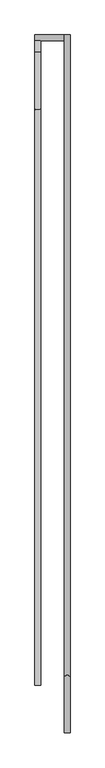
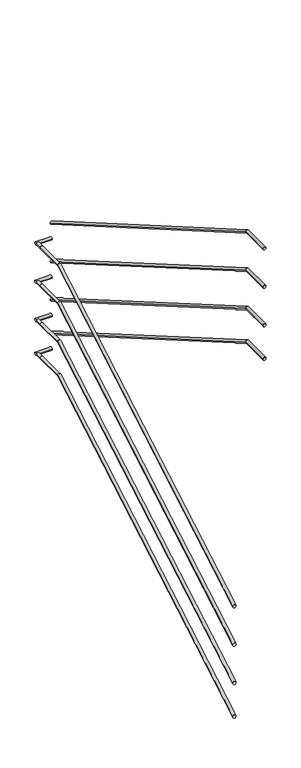
"""IFC4 building model written with IfcOpenShell, lengths in millimetres: railing geometry."""

from ifc_helpers import new_model, si_unit, frame, origin, place, context, project, spatial, circle_curve, ellipse_curve, source, transform, mapped, element, save
from ifc_brep_helpers import plane_surface, cylinder_surface, advanced_brep


def railing_01d63982(model_context):
    return source(origin(), model_context, "Body", "AdvancedBrep", [
        advanced_brep(
        [(52769.6, 12029.5208589, 12766.5366726), (52799.6, 12029.5208589, 12766.5366726), (52769.6, 15033.554313, 14508.0053416), (52799.6, 15033.554313, 14508.0053416), (52769.6, 15329.5208589, 14508.0053416), (52799.6, 15329.5208589, 14508.0053416)],
        [
            (0, 1, ellipse_curve(frame((52784.6, 12029.5208589, 12766.5366726), z_axis=(0.0, -1.0, 0.0), x_axis=(0.0, 0.0, -1.0)), 17.3382342, 15.0)),
            (1, 0, ellipse_curve(frame((52784.6, 12029.5208589, 12766.5366726), z_axis=(0.0, -1.0, 0.0), x_axis=(0.0, 0.0, -1.0)), 17.3382342, 15.0)),
            (0, 2),
            (2, 3, ellipse_curve(frame((52784.6, 15033.554313, 14508.0053416), z_axis=(0.0, -0.9656966401166088, -0.25967286971782944), x_axis=(0.0, 0.25967286971782905, -0.9656966401166089)), 15.5328282, 15.0)),
            (3, 1),
            (3, 2, ellipse_curve(frame((52784.6, 15033.554313, 14508.0053416), z_axis=(0.0, -0.9656966401166088, -0.25967286971782944), x_axis=(0.0, 0.25967286971782905, -0.9656966401166089)), 15.5328282, 15.0)),
            (4, 5, circle_curve(frame((52784.6, 15329.5208589, 14508.0053416), z_axis=(0.0, 1.0, 0.0), x_axis=(1.0, 0.0, 0.0)), 15.0)),
            (5, 4, circle_curve(frame((52784.6, 15329.5208589, 14508.0053416), z_axis=(0.0, 1.0, 0.0), x_axis=(1.0, 0.0, 0.0)), 15.0)),
            (2, 4),
            (5, 3),
        ],
        [
            plane_surface(frame((52784.6, 12029.5208589, 12783.8749068), z_axis=(0.0, -1.0, 0.0), x_axis=(0.0, 0.0, 1.0))),
            cylinder_surface(frame((52784.6, 12037.0438154, 12770.8978068), z_axis=(0.0, -0.8651400014650144, -0.5015304356318916), x_axis=(1.0, 0.0, 0.0)), 15.0),
            plane_surface(frame((52784.6, 15329.5208589, 14523.0053416), z_axis=(0.0, 1.0, 0.0), x_axis=(0.0, 0.0, 1.0))),
            cylinder_surface(frame((52784.6, 15029.5208589, 14508.0053416), z_axis=(0.0, -1.0, 0.0), x_axis=(1.0, 0.0, 0.0)), 15.0),
        ],
        [
            (0, [[1, 2]]),
            (1, [[-1, 3, 4, 5]]),
            (1, [[-2, -5, 6, -3]]),
            (2, [[7, 8]]),
            (3, [[-4, 9, -8, 10]]),
            (3, [[-6, -10, -7, -9]]),
        ],
    ),
        advanced_brep(
        [(52769.6, 15329.5208589, 14508.0053416), (52799.6, 15329.5208589, 14508.0053416), (52769.6, 15389.9208589, 14508.0053416), (52799.6, 15389.9208589, 14508.0053416)],
        [
            (0, 1, circle_curve(frame((52784.6, 15329.5208589, 14508.0053416), z_axis=(0.0, -1.0, 0.0), x_axis=(1.0, 0.0, 0.0)), 15.0)),
            (1, 0, circle_curve(frame((52784.6, 15329.5208589, 14508.0053416), z_axis=(0.0, -1.0, 0.0), x_axis=(1.0, 0.0, 0.0)), 15.0)),
            (2, 3, circle_curve(frame((52784.6, 15389.9208589, 14508.0053416), z_axis=(0.0, 1.0, 0.0), x_axis=(1.0, 0.0, 0.0)), 15.0)),
            (3, 2, circle_curve(frame((52784.6, 15389.9208589, 14508.0053416), z_axis=(0.0, 1.0, 0.0), x_axis=(1.0, 0.0, 0.0)), 15.0)),
            (0, 2),
            (3, 1),
        ],
        [
            plane_surface(frame((52784.6, 15329.5208589, 14523.0053416), z_axis=(0.0, -1.0, 0.0), x_axis=(0.0, 0.0, 1.0))),
            plane_surface(frame((52784.6, 15389.9208589, 14523.0053416), z_axis=(0.0, 1.0, 0.0), x_axis=(0.0, 0.0, 1.0))),
            cylinder_surface(frame((52784.6, 15329.5208589, 14508.0053416), z_axis=(0.0, -1.0, 0.0), x_axis=(1.0, 0.0, 0.0)), 15.0),
        ],
        [
            (0, [[1, 2]]),
            (1, [[3, 4]]),
            (2, [[-1, 5, -4, 6]]),
            (2, [[-2, -6, -3, -5]]),
        ],
    ),
        advanced_brep(
        [(52769.6, 15419.9208589, 14508.0053416), (52769.6, 15389.9208589, 14508.0053416), (52922.635546, 15419.9208589, 14508.0053416), (52922.635546, 15389.9208589, 14508.0053416)],
        [
            (0, 1, circle_curve(frame((52769.6, 15404.9208589, 14508.0053416), z_axis=(-1.0, 0.0, 0.0), x_axis=(0.0, -1.0, 0.0)), 15.0)),
            (1, 0, circle_curve(frame((52769.6, 15404.9208589, 14508.0053416), z_axis=(-1.0, 0.0, 0.0), x_axis=(0.0, -1.0, 0.0)), 15.0)),
            (2, 3, circle_curve(frame((52922.635546, 15404.9208589, 14508.0053416), z_axis=(1.0, 0.0, 0.0), x_axis=(0.0, -1.0, 0.0)), 15.0)),
            (3, 2, circle_curve(frame((52922.635546, 15404.9208589, 14508.0053416), z_axis=(1.0, 0.0, 0.0), x_axis=(0.0, -1.0, 0.0)), 15.0)),
            (0, 2),
            (3, 1),
        ],
        [
            plane_surface(frame((52769.6, 15404.9208589, 14523.0053416), z_axis=(-1.0, 0.0, 0.0), x_axis=(0.0, 1.0, 0.0))),
            plane_surface(frame((52922.635546, 15404.9208589, 14523.0053416), z_axis=(1.0, 0.0, 0.0), x_axis=(0.0, 1.0, 0.0))),
            cylinder_surface(frame((52769.6, 15404.9208589, 14508.0053416), z_axis=(-1.0, 0.0, 0.0), x_axis=(0.0, -1.0, 0.0)), 15.0),
        ],
        [
            (0, [[1, 2]]),
            (1, [[3, 4]]),
            (2, [[-1, 5, -4, 6]]),
            (2, [[-2, -6, -3, -5]]),
        ],
    ),
        advanced_brep(
        [(52952.635546, 15419.9208589, 14656.159861), (52922.635546, 15419.9208589, 14656.159861), (52952.635546, 12075.4874048, 16594.9618634), (52922.635546, 12075.4874048, 16594.9618634), (52952.635546, 11779.5208589, 16594.9618634), (52922.635546, 11779.5208589, 16594.9618634)],
        [
            (0, 1, ellipse_curve(frame((52937.635546, 15419.9208589, 14656.159861), z_axis=(0.0, 1.0, 0.0), x_axis=(0.0, 0.0, -1.0)), 17.3382342, 15.0)),
            (1, 0, ellipse_curve(frame((52937.635546, 15419.9208589, 14656.159861), z_axis=(0.0, 1.0, 0.0), x_axis=(0.0, 0.0, -1.0)), 17.3382342, 15.0)),
            (0, 2),
            (2, 3, ellipse_curve(frame((52937.635546, 12075.4874048, 16594.9618634), z_axis=(0.0, 0.9656966401166087, -0.2596728697178297), x_axis=(0.0, -0.259672869717829, -0.9656966401166089)), 15.5328282, 15.0)),
            (3, 1),
            (3, 2, ellipse_curve(frame((52937.635546, 12075.4874048, 16594.9618634), z_axis=(0.0, 0.9656966401166087, -0.2596728697178297), x_axis=(0.0, -0.259672869717829, -0.9656966401166089)), 15.5328282, 15.0)),
            (4, 5, circle_curve(frame((52937.635546, 11779.5208589, 16594.9618634), z_axis=(0.0, -1.0, 0.0), x_axis=(-1.0, 0.0, 0.0)), 15.0)),
            (5, 4, circle_curve(frame((52937.635546, 11779.5208589, 16594.9618634), z_axis=(0.0, -1.0, 0.0), x_axis=(-1.0, 0.0, 0.0)), 15.0)),
            (2, 4),
            (5, 3),
        ],
        [
            plane_surface(frame((52937.635546, 15419.9208589, 14673.4980953), z_axis=(0.0, 1.0, 0.0), x_axis=(0.0, 0.0, -1.0))),
            cylinder_surface(frame((52937.635546, 15412.3979024, 14660.5209952), z_axis=(0.0, 0.865140001465014, -0.5015304356318923), x_axis=(-1.0, 0.0, 0.0)), 15.0),
            plane_surface(frame((52937.635546, 11779.5208589, 16609.9618634), z_axis=(0.0, -1.0, 0.0), x_axis=(0.0, 0.0, -1.0))),
            cylinder_surface(frame((52937.635546, 12079.5208589, 16594.9618634), z_axis=(0.0, 1.0, 0.0), x_axis=(-1.0, 0.0, 0.0)), 15.0),
        ],
        [
            (0, [[1, 2]]),
            (1, [[-1, 3, 4, 5]]),
            (1, [[-2, -5, 6, -3]]),
            (2, [[7, 8]]),
            (3, [[-4, 9, -8, 10]]),
            (3, [[-6, -10, -7, -9]]),
        ],
    ),
        advanced_brep(
        [(52769.6, 12029.5208589, 11966.5366726), (52799.6, 12029.5208589, 11966.5366726), (52769.6, 15033.554313, 13708.0053416), (52799.6, 15033.554313, 13708.0053416), (52769.6, 15329.5208589, 13708.0053416), (52799.6, 15329.5208589, 13708.0053416)],
        [
            (0, 1, ellipse_curve(frame((52784.6, 12029.5208589, 11966.5366726), z_axis=(0.0, -1.0, 0.0), x_axis=(0.0, 0.0, -1.0)), 17.3382342, 15.0)),
            (1, 0, ellipse_curve(frame((52784.6, 12029.5208589, 11966.5366726), z_axis=(0.0, -1.0, 0.0), x_axis=(0.0, 0.0, -1.0)), 17.3382342, 15.0)),
            (0, 2),
            (2, 3, ellipse_curve(frame((52784.6, 15033.554313, 13708.0053416), z_axis=(0.0, -0.9656966401166088, -0.25967286971782944), x_axis=(0.0, 0.25967286971782905, -0.9656966401166089)), 15.5328282, 15.0)),
            (3, 1),
            (3, 2, ellipse_curve(frame((52784.6, 15033.554313, 13708.0053416), z_axis=(0.0, -0.9656966401166088, -0.25967286971782944), x_axis=(0.0, 0.25967286971782905, -0.9656966401166089)), 15.5328282, 15.0)),
            (4, 5, circle_curve(frame((52784.6, 15329.5208589, 13708.0053416), z_axis=(0.0, 1.0, 0.0), x_axis=(1.0, 0.0, 0.0)), 15.0)),
            (5, 4, circle_curve(frame((52784.6, 15329.5208589, 13708.0053416), z_axis=(0.0, 1.0, 0.0), x_axis=(1.0, 0.0, 0.0)), 15.0)),
            (2, 4),
            (5, 3),
        ],
        [
            plane_surface(frame((52784.6, 12029.5208589, 11983.8749068), z_axis=(0.0, -1.0, 0.0), x_axis=(0.0, 0.0, 1.0))),
            cylinder_surface(frame((52784.6, 12037.0438154, 11970.8978068), z_axis=(0.0, -0.8651400014650144, -0.5015304356318916), x_axis=(1.0, 0.0, 0.0)), 15.0),
            plane_surface(frame((52784.6, 15329.5208589, 13723.0053416), z_axis=(0.0, 1.0, 0.0), x_axis=(0.0, 0.0, 1.0))),
            cylinder_surface(frame((52784.6, 15029.5208589, 13708.0053416), z_axis=(0.0, -1.0, 0.0), x_axis=(1.0, 0.0, 0.0)), 15.0),
        ],
        [
            (0, [[1, 2]]),
            (1, [[-1, 3, 4, 5]]),
            (1, [[-2, -5, 6, -3]]),
            (2, [[7, 8]]),
            (3, [[-4, 9, -8, 10]]),
            (3, [[-6, -10, -7, -9]]),
        ],
    ),
        advanced_brep(
        [(52769.6, 15329.5208589, 13708.0053416), (52799.6, 15329.5208589, 13708.0053416), (52769.6, 15389.9208589, 13708.0053416), (52799.6, 15389.9208589, 13708.0053416)],
        [
            (0, 1, circle_curve(frame((52784.6, 15329.5208589, 13708.0053416), z_axis=(0.0, -1.0, 0.0), x_axis=(1.0, 0.0, 0.0)), 15.0)),
            (1, 0, circle_curve(frame((52784.6, 15329.5208589, 13708.0053416), z_axis=(0.0, -1.0, 0.0), x_axis=(1.0, 0.0, 0.0)), 15.0)),
            (2, 3, circle_curve(frame((52784.6, 15389.9208589, 13708.0053416), z_axis=(0.0, 1.0, 0.0), x_axis=(1.0, 0.0, 0.0)), 15.0)),
            (3, 2, circle_curve(frame((52784.6, 15389.9208589, 13708.0053416), z_axis=(0.0, 1.0, 0.0), x_axis=(1.0, 0.0, 0.0)), 15.0)),
            (0, 2),
            (3, 1),
        ],
        [
            plane_surface(frame((52784.6, 15329.5208589, 13723.0053416), z_axis=(0.0, -1.0, 0.0), x_axis=(0.0, 0.0, 1.0))),
            plane_surface(frame((52784.6, 15389.9208589, 13723.0053416), z_axis=(0.0, 1.0, 0.0), x_axis=(0.0, 0.0, 1.0))),
            cylinder_surface(frame((52784.6, 15329.5208589, 13708.0053416), z_axis=(0.0, -1.0, 0.0), x_axis=(1.0, 0.0, 0.0)), 15.0),
        ],
        [
            (0, [[1, 2]]),
            (1, [[3, 4]]),
            (2, [[-1, 5, -4, 6]]),
            (2, [[-2, -6, -3, -5]]),
        ],
    ),
        advanced_brep(
        [(52769.6, 15419.9208589, 13708.0053416), (52769.6, 15389.9208589, 13708.0053416), (52922.635546, 15419.9208589, 13708.0053416), (52922.635546, 15389.9208589, 13708.0053416)],
        [
            (0, 1, circle_curve(frame((52769.6, 15404.9208589, 13708.0053416), z_axis=(-1.0, 0.0, 0.0), x_axis=(0.0, -1.0, 0.0)), 15.0)),
            (1, 0, circle_curve(frame((52769.6, 15404.9208589, 13708.0053416), z_axis=(-1.0, 0.0, 0.0), x_axis=(0.0, -1.0, 0.0)), 15.0)),
            (2, 3, circle_curve(frame((52922.635546, 15404.9208589, 13708.0053416), z_axis=(1.0, 0.0, 0.0), x_axis=(0.0, -1.0, 0.0)), 15.0)),
            (3, 2, circle_curve(frame((52922.635546, 15404.9208589, 13708.0053416), z_axis=(1.0, 0.0, 0.0), x_axis=(0.0, -1.0, 0.0)), 15.0)),
            (0, 2),
            (3, 1),
        ],
        [
            plane_surface(frame((52769.6, 15404.9208589, 13723.0053416), z_axis=(-1.0, 0.0, 0.0), x_axis=(0.0, 1.0, 0.0))),
            plane_surface(frame((52922.635546, 15404.9208589, 13723.0053416), z_axis=(1.0, 0.0, 0.0), x_axis=(0.0, 1.0, 0.0))),
            cylinder_surface(frame((52769.6, 15404.9208589, 13708.0053416), z_axis=(-1.0, 0.0, 0.0), x_axis=(0.0, -1.0, 0.0)), 15.0),
        ],
        [
            (0, [[1, 2]]),
            (1, [[3, 4]]),
            (2, [[-1, 5, -4, 6]]),
            (2, [[-2, -6, -3, -5]]),
        ],
    ),
        advanced_brep(
        [(52952.635546, 15419.9208589, 13856.159861), (52922.635546, 15419.9208589, 13856.159861), (52952.635546, 12075.4874048, 15794.9618634), (52922.635546, 12075.4874048, 15794.9618634), (52952.635546, 11779.5208589, 15794.9618634), (52922.635546, 11779.5208589, 15794.9618634)],
        [
            (0, 1, ellipse_curve(frame((52937.635546, 15419.9208589, 13856.159861), z_axis=(0.0, 1.0, 0.0), x_axis=(0.0, 0.0, -1.0)), 17.3382342, 15.0)),
            (1, 0, ellipse_curve(frame((52937.635546, 15419.9208589, 13856.159861), z_axis=(0.0, 1.0, 0.0), x_axis=(0.0, 0.0, -1.0)), 17.3382342, 15.0)),
            (0, 2),
            (2, 3, ellipse_curve(frame((52937.635546, 12075.4874048, 15794.9618634), z_axis=(0.0, 0.9656966401166087, -0.2596728697178297), x_axis=(0.0, -0.259672869717829, -0.9656966401166089)), 15.5328282, 15.0)),
            (3, 1),
            (3, 2, ellipse_curve(frame((52937.635546, 12075.4874048, 15794.9618634), z_axis=(0.0, 0.9656966401166087, -0.2596728697178297), x_axis=(0.0, -0.259672869717829, -0.9656966401166089)), 15.5328282, 15.0)),
            (4, 5, circle_curve(frame((52937.635546, 11779.5208589, 15794.9618634), z_axis=(0.0, -1.0, 0.0), x_axis=(-1.0, 0.0, 0.0)), 15.0)),
            (5, 4, circle_curve(frame((52937.635546, 11779.5208589, 15794.9618634), z_axis=(0.0, -1.0, 0.0), x_axis=(-1.0, 0.0, 0.0)), 15.0)),
            (2, 4),
            (5, 3),
        ],
        [
            plane_surface(frame((52937.635546, 15419.9208589, 13873.4980953), z_axis=(0.0, 1.0, 0.0), x_axis=(0.0, 0.0, -1.0))),
            cylinder_surface(frame((52937.635546, 15412.3979024, 13860.5209952), z_axis=(0.0, 0.865140001465014, -0.5015304356318923), x_axis=(-1.0, 0.0, 0.0)), 15.0),
            plane_surface(frame((52937.635546, 11779.5208589, 15809.9618634), z_axis=(0.0, -1.0, 0.0), x_axis=(0.0, 0.0, -1.0))),
            cylinder_surface(frame((52937.635546, 12079.5208589, 15794.9618634), z_axis=(0.0, 1.0, 0.0), x_axis=(-1.0, 0.0, 0.0)), 15.0),
        ],
        [
            (0, [[1, 2]]),
            (1, [[-1, 3, 4, 5]]),
            (1, [[-2, -5, 6, -3]]),
            (2, [[7, 8]]),
            (3, [[-4, 9, -8, 10]]),
            (3, [[-6, -10, -7, -9]]),
        ],
    ),
        advanced_brep(
        [(52769.6, 12029.5208589, 12366.5366726), (52799.6, 12029.5208589, 12366.5366726), (52769.6, 15033.554313, 14108.0053416), (52799.6, 15033.554313, 14108.0053416), (52769.6, 15329.5208589, 14108.0053416), (52799.6, 15329.5208589, 14108.0053416)],
        [
            (0, 1, ellipse_curve(frame((52784.6, 12029.5208589, 12366.5366726), z_axis=(0.0, -1.0, 0.0), x_axis=(0.0, 0.0, -1.0)), 17.3382342, 15.0)),
            (1, 0, ellipse_curve(frame((52784.6, 12029.5208589, 12366.5366726), z_axis=(0.0, -1.0, 0.0), x_axis=(0.0, 0.0, -1.0)), 17.3382342, 15.0)),
            (0, 2),
            (2, 3, ellipse_curve(frame((52784.6, 15033.554313, 14108.0053416), z_axis=(0.0, -0.9656966401166088, -0.25967286971782944), x_axis=(0.0, 0.25967286971782905, -0.9656966401166089)), 15.5328282, 15.0)),
            (3, 1),
            (3, 2, ellipse_curve(frame((52784.6, 15033.554313, 14108.0053416), z_axis=(0.0, -0.9656966401166088, -0.25967286971782944), x_axis=(0.0, 0.25967286971782905, -0.9656966401166089)), 15.5328282, 15.0)),
            (4, 5, circle_curve(frame((52784.6, 15329.5208589, 14108.0053416), z_axis=(0.0, 1.0, 0.0), x_axis=(1.0, 0.0, 0.0)), 15.0)),
            (5, 4, circle_curve(frame((52784.6, 15329.5208589, 14108.0053416), z_axis=(0.0, 1.0, 0.0), x_axis=(1.0, 0.0, 0.0)), 15.0)),
            (2, 4),
            (5, 3),
        ],
        [
            plane_surface(frame((52784.6, 12029.5208589, 12383.8749068), z_axis=(0.0, -1.0, 0.0), x_axis=(0.0, 0.0, 1.0))),
            cylinder_surface(frame((52784.6, 12037.0438154, 12370.8978068), z_axis=(0.0, -0.8651400014650144, -0.5015304356318916), x_axis=(1.0, 0.0, 0.0)), 15.0),
            plane_surface(frame((52784.6, 15329.5208589, 14123.0053416), z_axis=(0.0, 1.0, 0.0), x_axis=(0.0, 0.0, 1.0))),
            cylinder_surface(frame((52784.6, 15029.5208589, 14108.0053416), z_axis=(0.0, -1.0, 0.0), x_axis=(1.0, 0.0, 0.0)), 15.0),
        ],
        [
            (0, [[1, 2]]),
            (1, [[-1, 3, 4, 5]]),
            (1, [[-2, -5, 6, -3]]),
            (2, [[7, 8]]),
            (3, [[-4, 9, -8, 10]]),
            (3, [[-6, -10, -7, -9]]),
        ],
    ),
        advanced_brep(
        [(52769.6, 15329.5208589, 14108.0053416), (52799.6, 15329.5208589, 14108.0053416), (52769.6, 15389.9208589, 14108.0053416), (52799.6, 15389.9208589, 14108.0053416)],
        [
            (0, 1, circle_curve(frame((52784.6, 15329.5208589, 14108.0053416), z_axis=(0.0, -1.0, 0.0), x_axis=(1.0, 0.0, 0.0)), 15.0)),
            (1, 0, circle_curve(frame((52784.6, 15329.5208589, 14108.0053416), z_axis=(0.0, -1.0, 0.0), x_axis=(1.0, 0.0, 0.0)), 15.0)),
            (2, 3, circle_curve(frame((52784.6, 15389.9208589, 14108.0053416), z_axis=(0.0, 1.0, 0.0), x_axis=(1.0, 0.0, 0.0)), 15.0)),
            (3, 2, circle_curve(frame((52784.6, 15389.9208589, 14108.0053416), z_axis=(0.0, 1.0, 0.0), x_axis=(1.0, 0.0, 0.0)), 15.0)),
            (0, 2),
            (3, 1),
        ],
        [
            plane_surface(frame((52784.6, 15329.5208589, 14123.0053416), z_axis=(0.0, -1.0, 0.0), x_axis=(0.0, 0.0, 1.0))),
            plane_surface(frame((52784.6, 15389.9208589, 14123.0053416), z_axis=(0.0, 1.0, 0.0), x_axis=(0.0, 0.0, 1.0))),
            cylinder_surface(frame((52784.6, 15329.5208589, 14108.0053416), z_axis=(0.0, -1.0, 0.0), x_axis=(1.0, 0.0, 0.0)), 15.0),
        ],
        [
            (0, [[1, 2]]),
            (1, [[3, 4]]),
            (2, [[-1, 5, -4, 6]]),
            (2, [[-2, -6, -3, -5]]),
        ],
    ),
        advanced_brep(
        [(52769.6, 15419.9208589, 14108.0053416), (52769.6, 15389.9208589, 14108.0053416), (52922.635546, 15419.9208589, 14108.0053416), (52922.635546, 15389.9208589, 14108.0053416)],
        [
            (0, 1, circle_curve(frame((52769.6, 15404.9208589, 14108.0053416), z_axis=(-1.0, 0.0, 0.0), x_axis=(0.0, -1.0, 0.0)), 15.0)),
            (1, 0, circle_curve(frame((52769.6, 15404.9208589, 14108.0053416), z_axis=(-1.0, 0.0, 0.0), x_axis=(0.0, -1.0, 0.0)), 15.0)),
            (2, 3, circle_curve(frame((52922.635546, 15404.9208589, 14108.0053416), z_axis=(1.0, 0.0, 0.0), x_axis=(0.0, -1.0, 0.0)), 15.0)),
            (3, 2, circle_curve(frame((52922.635546, 15404.9208589, 14108.0053416), z_axis=(1.0, 0.0, 0.0), x_axis=(0.0, -1.0, 0.0)), 15.0)),
            (0, 2),
            (3, 1),
        ],
        [
            plane_surface(frame((52769.6, 15404.9208589, 14123.0053416), z_axis=(-1.0, 0.0, 0.0), x_axis=(0.0, 1.0, 0.0))),
            plane_surface(frame((52922.635546, 15404.9208589, 14123.0053416), z_axis=(1.0, 0.0, 0.0), x_axis=(0.0, 1.0, 0.0))),
            cylinder_surface(frame((52769.6, 15404.9208589, 14108.0053416), z_axis=(-1.0, 0.0, 0.0), x_axis=(0.0, -1.0, 0.0)), 15.0),
        ],
        [
            (0, [[1, 2]]),
            (1, [[3, 4]]),
            (2, [[-1, 5, -4, 6]]),
            (2, [[-2, -6, -3, -5]]),
        ],
    ),
        advanced_brep(
        [(52952.635546, 15419.9208589, 14256.159861), (52922.635546, 15419.9208589, 14256.159861), (52952.635546, 12075.4874048, 16194.9618634), (52922.635546, 12075.4874048, 16194.9618634), (52952.635546, 11779.5208589, 16194.9618634), (52922.635546, 11779.5208589, 16194.9618634)],
        [
            (0, 1, ellipse_curve(frame((52937.635546, 15419.9208589, 14256.159861), z_axis=(0.0, 1.0, 0.0), x_axis=(0.0, 0.0, -1.0)), 17.3382342, 15.0)),
            (1, 0, ellipse_curve(frame((52937.635546, 15419.9208589, 14256.159861), z_axis=(0.0, 1.0, 0.0), x_axis=(0.0, 0.0, -1.0)), 17.3382342, 15.0)),
            (0, 2),
            (2, 3, ellipse_curve(frame((52937.635546, 12075.4874048, 16194.9618634), z_axis=(0.0, 0.9656966401166087, -0.2596728697178297), x_axis=(0.0, -0.259672869717829, -0.9656966401166089)), 15.5328282, 15.0)),
            (3, 1),
            (3, 2, ellipse_curve(frame((52937.635546, 12075.4874048, 16194.9618634), z_axis=(0.0, 0.9656966401166087, -0.2596728697178297), x_axis=(0.0, -0.259672869717829, -0.9656966401166089)), 15.5328282, 15.0)),
            (4, 5, circle_curve(frame((52937.635546, 11779.5208589, 16194.9618634), z_axis=(0.0, -1.0, 0.0), x_axis=(-1.0, 0.0, 0.0)), 15.0)),
            (5, 4, circle_curve(frame((52937.635546, 11779.5208589, 16194.9618634), z_axis=(0.0, -1.0, 0.0), x_axis=(-1.0, 0.0, 0.0)), 15.0)),
            (2, 4),
            (5, 3),
        ],
        [
            plane_surface(frame((52937.635546, 15419.9208589, 14273.4980953), z_axis=(0.0, 1.0, 0.0), x_axis=(0.0, 0.0, -1.0))),
            cylinder_surface(frame((52937.635546, 15412.3979024, 14260.5209952), z_axis=(0.0, 0.865140001465014, -0.5015304356318923), x_axis=(-1.0, 0.0, 0.0)), 15.0),
            plane_surface(frame((52937.635546, 11779.5208589, 16209.9618634), z_axis=(0.0, -1.0, 0.0), x_axis=(0.0, 0.0, -1.0))),
            cylinder_surface(frame((52937.635546, 12079.5208589, 16194.9618634), z_axis=(0.0, 1.0, 0.0), x_axis=(-1.0, 0.0, 0.0)), 15.0),
        ],
        [
            (0, [[1, 2]]),
            (1, [[-1, 3, 4, 5]]),
            (1, [[-2, -5, 6, -3]]),
            (2, [[7, 8]]),
            (3, [[-4, 9, -8, 10]]),
            (3, [[-6, -10, -7, -9]]),
        ],
    ),
        advanced_brep(
        [(52769.6, 12029.5208589, 11616.5366726), (52799.6, 12029.5208589, 11616.5366726), (52769.6, 15033.554313, 13358.0053416), (52799.6, 15033.554313, 13358.0053416), (52769.6, 15329.5208589, 13358.0053416), (52799.6, 15329.5208589, 13358.0053416)],
        [
            (0, 1, ellipse_curve(frame((52784.6, 12029.5208589, 11616.5366726), z_axis=(0.0, -1.0, 0.0), x_axis=(0.0, 0.0, -1.0)), 17.3382342, 15.0)),
            (1, 0, ellipse_curve(frame((52784.6, 12029.5208589, 11616.5366726), z_axis=(0.0, -1.0, 0.0), x_axis=(0.0, 0.0, -1.0)), 17.3382342, 15.0)),
            (0, 2),
            (2, 3, ellipse_curve(frame((52784.6, 15033.554313, 13358.0053416), z_axis=(0.0, -0.9656966401166088, -0.25967286971782944), x_axis=(0.0, 0.25967286971782905, -0.9656966401166089)), 15.5328282, 15.0)),
            (3, 1),
            (3, 2, ellipse_curve(frame((52784.6, 15033.554313, 13358.0053416), z_axis=(0.0, -0.9656966401166088, -0.25967286971782944), x_axis=(0.0, 0.25967286971782905, -0.9656966401166089)), 15.5328282, 15.0)),
            (4, 5, circle_curve(frame((52784.6, 15329.5208589, 13358.0053416), z_axis=(0.0, 1.0, 0.0), x_axis=(1.0, 0.0, 0.0)), 15.0)),
            (5, 4, circle_curve(frame((52784.6, 15329.5208589, 13358.0053416), z_axis=(0.0, 1.0, 0.0), x_axis=(1.0, 0.0, 0.0)), 15.0)),
            (2, 4),
            (5, 3),
        ],
        [
            plane_surface(frame((52784.6, 12029.5208589, 11633.8749068), z_axis=(0.0, -1.0, 0.0), x_axis=(0.0, 0.0, 1.0))),
            cylinder_surface(frame((52784.6, 12037.0438154, 11620.8978068), z_axis=(0.0, -0.8651400014650144, -0.5015304356318916), x_axis=(1.0, 0.0, 0.0)), 15.0),
            plane_surface(frame((52784.6, 15329.5208589, 13373.0053416), z_axis=(0.0, 1.0, 0.0), x_axis=(0.0, 0.0, 1.0))),
            cylinder_surface(frame((52784.6, 15029.5208589, 13358.0053416), z_axis=(0.0, -1.0, 0.0), x_axis=(1.0, 0.0, 0.0)), 15.0),
        ],
        [
            (0, [[1, 2]]),
            (1, [[-1, 3, 4, 5]]),
            (1, [[-2, -5, 6, -3]]),
            (2, [[7, 8]]),
            (3, [[-4, 9, -8, 10]]),
            (3, [[-6, -10, -7, -9]]),
        ],
    ),
        advanced_brep(
        [(52769.6, 15329.5208589, 13358.0053416), (52799.6, 15329.5208589, 13358.0053416), (52769.6, 15389.9208589, 13358.0053416), (52799.6, 15389.9208589, 13358.0053416)],
        [
            (0, 1, circle_curve(frame((52784.6, 15329.5208589, 13358.0053416), z_axis=(0.0, -1.0, 0.0), x_axis=(1.0, 0.0, 0.0)), 15.0)),
            (1, 0, circle_curve(frame((52784.6, 15329.5208589, 13358.0053416), z_axis=(0.0, -1.0, 0.0), x_axis=(1.0, 0.0, 0.0)), 15.0)),
            (2, 3, circle_curve(frame((52784.6, 15389.9208589, 13358.0053416), z_axis=(0.0, 1.0, 0.0), x_axis=(1.0, 0.0, 0.0)), 15.0)),
            (3, 2, circle_curve(frame((52784.6, 15389.9208589, 13358.0053416), z_axis=(0.0, 1.0, 0.0), x_axis=(1.0, 0.0, 0.0)), 15.0)),
            (0, 2),
            (3, 1),
        ],
        [
            plane_surface(frame((52784.6, 15329.5208589, 13373.0053416), z_axis=(0.0, -1.0, 0.0), x_axis=(0.0, 0.0, 1.0))),
            plane_surface(frame((52784.6, 15389.9208589, 13373.0053416), z_axis=(0.0, 1.0, 0.0), x_axis=(0.0, 0.0, 1.0))),
            cylinder_surface(frame((52784.6, 15329.5208589, 13358.0053416), z_axis=(0.0, -1.0, 0.0), x_axis=(1.0, 0.0, 0.0)), 15.0),
        ],
        [
            (0, [[1, 2]]),
            (1, [[3, 4]]),
            (2, [[-1, 5, -4, 6]]),
            (2, [[-2, -6, -3, -5]]),
        ],
    ),
        advanced_brep(
        [(52769.6, 15419.9208589, 13358.0053416), (52769.6, 15389.9208589, 13358.0053416), (52922.635546, 15419.9208589, 13358.0053416), (52922.635546, 15389.9208589, 13358.0053416)],
        [
            (0, 1, circle_curve(frame((52769.6, 15404.9208589, 13358.0053416), z_axis=(-1.0, 0.0, 0.0), x_axis=(0.0, -1.0, 0.0)), 15.0)),
            (1, 0, circle_curve(frame((52769.6, 15404.9208589, 13358.0053416), z_axis=(-1.0, 0.0, 0.0), x_axis=(0.0, -1.0, 0.0)), 15.0)),
            (2, 3, circle_curve(frame((52922.635546, 15404.9208589, 13358.0053416), z_axis=(1.0, 0.0, 0.0), x_axis=(0.0, -1.0, 0.0)), 15.0)),
            (3, 2, circle_curve(frame((52922.635546, 15404.9208589, 13358.0053416), z_axis=(1.0, 0.0, 0.0), x_axis=(0.0, -1.0, 0.0)), 15.0)),
            (0, 2),
            (3, 1),
        ],
        [
            plane_surface(frame((52769.6, 15404.9208589, 13373.0053416), z_axis=(-1.0, 0.0, 0.0), x_axis=(0.0, 1.0, 0.0))),
            plane_surface(frame((52922.635546, 15404.9208589, 13373.0053416), z_axis=(1.0, 0.0, 0.0), x_axis=(0.0, 1.0, 0.0))),
            cylinder_surface(frame((52769.6, 15404.9208589, 13358.0053416), z_axis=(-1.0, 0.0, 0.0), x_axis=(0.0, -1.0, 0.0)), 15.0),
        ],
        [
            (0, [[1, 2]]),
            (1, [[3, 4]]),
            (2, [[-1, 5, -4, 6]]),
            (2, [[-2, -6, -3, -5]]),
        ],
    ),
        advanced_brep(
        [(52952.635546, 15419.9208589, 13506.159861), (52922.635546, 15419.9208589, 13506.159861), (52952.635546, 12075.4874048, 15444.9618634), (52922.635546, 12075.4874048, 15444.9618634), (52952.635546, 11779.5208589, 15444.9618634), (52922.635546, 11779.5208589, 15444.9618634)],
        [
            (0, 1, ellipse_curve(frame((52937.635546, 15419.9208589, 13506.159861), z_axis=(0.0, 1.0, 0.0), x_axis=(0.0, 0.0, -1.0)), 17.3382342, 15.0)),
            (1, 0, ellipse_curve(frame((52937.635546, 15419.9208589, 13506.159861), z_axis=(0.0, 1.0, 0.0), x_axis=(0.0, 0.0, -1.0)), 17.3382342, 15.0)),
            (0, 2),
            (2, 3, ellipse_curve(frame((52937.635546, 12075.4874048, 15444.9618634), z_axis=(0.0, 0.9656966401166087, -0.2596728697178297), x_axis=(0.0, -0.259672869717829, -0.9656966401166089)), 15.5328282, 15.0)),
            (3, 1),
            (3, 2, ellipse_curve(frame((52937.635546, 12075.4874048, 15444.9618634), z_axis=(0.0, 0.9656966401166087, -0.2596728697178297), x_axis=(0.0, -0.259672869717829, -0.9656966401166089)), 15.5328282, 15.0)),
            (4, 5, circle_curve(frame((52937.635546, 11779.5208589, 15444.9618634), z_axis=(0.0, -1.0, 0.0), x_axis=(-1.0, 0.0, 0.0)), 15.0)),
            (5, 4, circle_curve(frame((52937.635546, 11779.5208589, 15444.9618634), z_axis=(0.0, -1.0, 0.0), x_axis=(-1.0, 0.0, 0.0)), 15.0)),
            (2, 4),
            (5, 3),
        ],
        [
            plane_surface(frame((52937.635546, 15419.9208589, 13523.4980953), z_axis=(0.0, 1.0, 0.0), x_axis=(0.0, 0.0, -1.0))),
            cylinder_surface(frame((52937.635546, 15412.3979024, 13510.5209952), z_axis=(0.0, 0.865140001465014, -0.5015304356318923), x_axis=(-1.0, 0.0, 0.0)), 15.0),
            plane_surface(frame((52937.635546, 11779.5208589, 15459.9618634), z_axis=(0.0, -1.0, 0.0), x_axis=(0.0, 0.0, -1.0))),
            cylinder_surface(frame((52937.635546, 12079.5208589, 15444.9618634), z_axis=(0.0, 1.0, 0.0), x_axis=(-1.0, 0.0, 0.0)), 15.0),
        ],
        [
            (0, [[1, 2]]),
            (1, [[-1, 3, 4, 5]]),
            (1, [[-2, -5, 6, -3]]),
            (2, [[7, 8]]),
            (3, [[-4, 9, -8, 10]]),
            (3, [[-6, -10, -7, -9]]),
        ],
    ),
    ])


if __name__ == "__main__":
    model = new_model("IFC4")
    model_context = context("Model", 3, world=origin())
    ifc_project = project(units=[si_unit("LENGTHUNIT", "METRE", prefix="MILLI")], contexts=[model_context])
    site = spatial("IfcSite", under=ifc_project)
    building = spatial("IfcBuilding", under=site)
    placement = place(None, origin())
    railing_shape = railing_01d63982(model_context)
    element("IfcRailing", 1, at=placement, inside=building, context=model_context, shape_type="MappedRepresentation", body=[
        mapped(railing_shape, transform((0.0, 0.0, 0.0), x_axis=(1.0, 0.0, 0.0), y_axis=(0.0, 1.0, 0.0), z_axis=(0.0, 0.0, 1.0))),
    ])
    save(model, "model.ifc")
